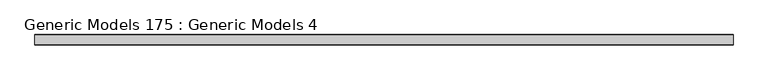
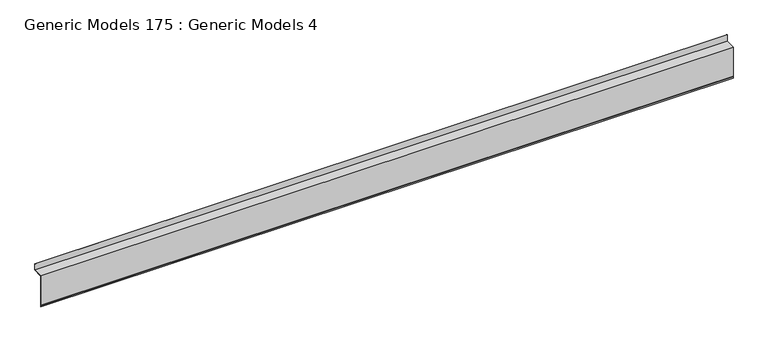
"""IFC4 building model written with IfcOpenShell, lengths in millimetres: proxy geometry, Generic Models 175 : Generic Models 4."""

from ifc_helpers import new_model, si_unit, frame, origin, place, context, project, spatial, polyline, outline, extrude, source, transform, mapped, element, save


def generic_models_175_generic_models_4_a406fa1a(model_context):
    return source(origin(), model_context, "Body", "SweptSolid", [
        extrude(outline(polyline([(-5649.1440684, 126372.71972), (-5649.1440684, 126346.9628262), (-5649.9378184, 126346.9628262), (-5649.9378184, 126372.8596795), (-5647.3420044, 126379.9916201), (-5647.3420044, 126931.9333762), (-5468.6027337, 126939.3808458), (-5468.6027337, 127056.8429876), (-5467.8089837, 127056.8429876), (-5467.8089837, 126938.61948), (-5646.5482544, 126931.1720104), (-5646.5482544, 126379.8516605), (-5649.1440684, 126372.71972)])), frame((-10234.5171316, 0.0, 0.0), z_axis=(1.0, 0.0, 0.0), x_axis=(0.0, 1.0, 0.0)), (0.0, 0.0, 1.0), 12431.443502),
    ])


if __name__ == "__main__":
    model = new_model("IFC4")
    model_context = context("Model", 3, world=origin())
    ifc_project = project(units=[si_unit("LENGTHUNIT", "METRE", prefix="MILLI")], contexts=[model_context])
    site = spatial("IfcSite", under=ifc_project)
    building = spatial("IfcBuilding", under=site)
    placement = place(None, origin())
    generic_models_175_generic_models_4_shape = generic_models_175_generic_models_4_a406fa1a(model_context)
    element("IfcBuildingElementProxy", 1, Name="Generic Models 175 : Generic Models 4", ObjectType="Generic Models 175 : Generic Models 4", at=placement, inside=building, context=model_context, shape_type="MappedRepresentation", body=[
        mapped(generic_models_175_generic_models_4_shape, transform((0.0, 0.0, 0.0), x_axis=(1.0, 0.0, 0.0), y_axis=(0.0, 1.0, 0.0), z_axis=(0.0, 0.0, 1.0))),
    ])
    save(model, "model.ifc")

# Revit data of these elements
# Element 1 (IfcBuildingElementProxy, "Generic Models 175 : Generic Models 4")
#   Materials on its faces: "_(2) LAYERS NO. 30 ASTM D226 ASPHALT SATURATED ORGANIC FELT"
# Materials
#   "_(2) LAYERS NO. 30 ASTM D226 ASPHALT SATURATED ORGANIC FELT": class "Generic", colour RGB 67 154 161, transparency 0, Cost = 0
